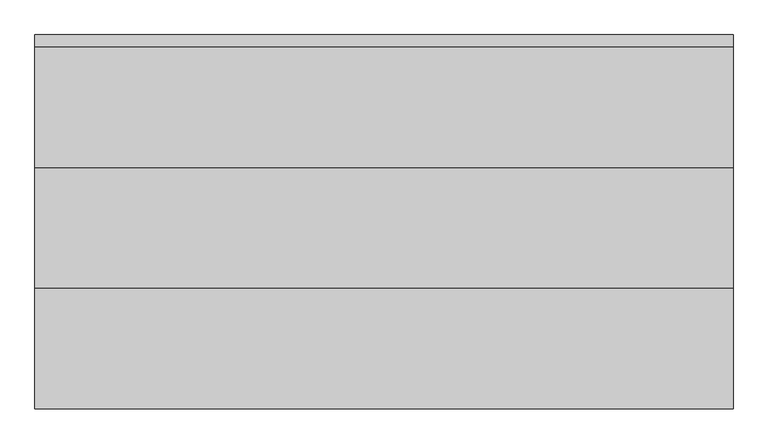
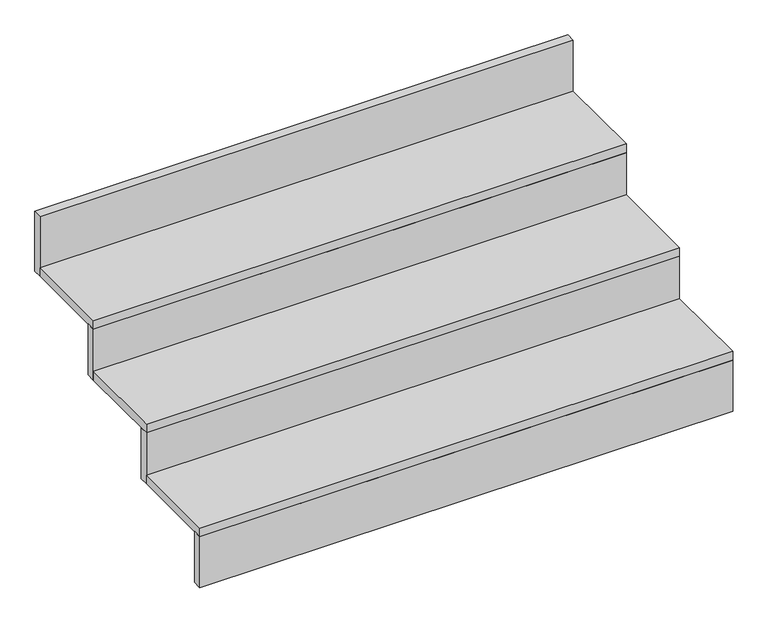
"""IFC4 building model written with IfcOpenShell, lengths in millimetres: stair flight geometry."""

from ifc_helpers import new_model, si_unit, frame, origin, place, context, project, spatial, polyline, outline, extrude, source, transform, mapped, element, save


def stair_flight_d92d106e(model_context):
    return source(origin(), model_context, "Body", "SweptSolid", [
        extrude(outline(polyline([(52810.0, -4270.0), (52810.0, -4300.0), (51075.0, -4300.0), (51075.0, -4270.0), (52810.0, -4270.0)])), frame((0.0, 0.0, 14070.0), z_axis=(0.0, 0.0, 1.0), x_axis=(1.0, 0.0, 0.0)), (0.0, 0.0, 1.0), 175.0),
        extrude(outline(polyline([(51075.0, -4000.0), (52810.0, -4000.0), (52810.0, -4300.0), (51075.0, -4300.0), (51075.0, -4000.0)])), frame((0.0, 0.0, 14245.0), z_axis=(0.0, 0.0, 1.0), x_axis=(1.0, 0.0, 0.0)), (0.0, 0.0, 1.0), 30.0),
        extrude(outline(polyline([(52810.0, -3970.0), (52810.0, -4000.0), (51075.0, -4000.0), (51075.0, -3970.0), (52810.0, -3970.0)])), frame((0.0, 0.0, 14245.0), z_axis=(0.0, 0.0, 1.0), x_axis=(1.0, 0.0, 0.0)), (0.0, 0.0, 1.0), 175.0),
        extrude(outline(polyline([(51075.0, -3700.0), (52810.0, -3700.0), (52810.0, -4000.0), (51075.0, -4000.0), (51075.0, -3700.0)])), frame((0.0, 0.0, 14420.0), z_axis=(0.0, 0.0, 1.0), x_axis=(1.0, 0.0, 0.0)), (0.0, 0.0, 1.0), 30.0),
        extrude(outline(polyline([(52810.0, -3670.0), (52810.0, -3700.0), (51075.0, -3700.0), (51075.0, -3670.0), (52810.0, -3670.0)])), frame((0.0, 0.0, 14420.0), z_axis=(0.0, 0.0, 1.0), x_axis=(1.0, 0.0, 0.0)), (0.0, 0.0, 1.0), 175.0),
        extrude(outline(polyline([(51075.0, -3400.0), (52810.0, -3400.0), (52810.0, -3700.0), (51075.0, -3700.0), (51075.0, -3400.0)])), frame((0.0, 0.0, 14595.0), z_axis=(0.0, 0.0, 1.0), x_axis=(1.0, 0.0, 0.0)), (0.0, 0.0, 1.0), 30.0),
        extrude(outline(polyline([(52810.0, -3370.0), (52810.0, -3400.0), (51075.0, -3400.0), (51075.0, -3370.0), (52810.0, -3370.0)])), frame((0.0, 0.0, 14595.0), z_axis=(0.0, 0.0, 1.0), x_axis=(1.0, 0.0, 0.0)), (0.0, 0.0, 1.0), 205.0),
    ])


if __name__ == "__main__":
    model = new_model("IFC4")
    model_context = context("Model", 3, world=origin())
    ifc_project = project(units=[si_unit("LENGTHUNIT", "METRE", prefix="MILLI")], contexts=[model_context])
    site = spatial("IfcSite", under=ifc_project)
    building = spatial("IfcBuilding", under=site)
    placement = place(None, origin())
    stair_flight_shape = stair_flight_d92d106e(model_context)
    element("IfcStairFlight", 1, at=placement, inside=building, context=model_context, shape_type="MappedRepresentation", body=[
        mapped(stair_flight_shape, transform((0.0, 0.0, 0.0), x_axis=(1.0, 0.0, 0.0), y_axis=(0.0, 1.0, 0.0), z_axis=(0.0, 0.0, 1.0))),
    ])
    save(model, "model.ifc")

# Revit data of these elements
# Element 1 (IfcStairFlight)
#   Materials on its faces: "00_Finish_Deco Tile"
# Materials
#   "00_Finish_Deco Tile": class "Finish", colour RGB 245 245 245, transparency 0, Description = "Ceramic Tile", Cost = 0
